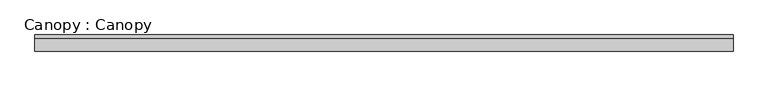
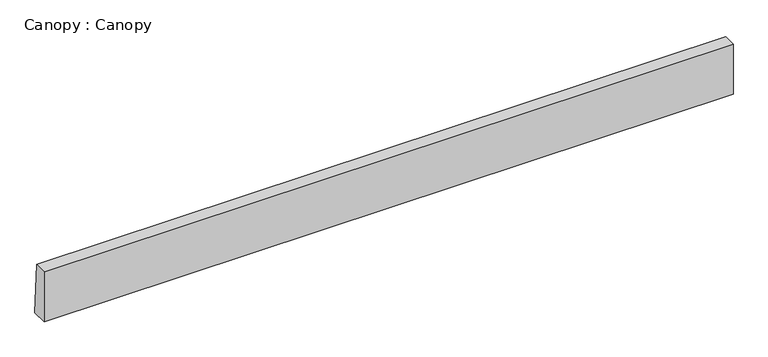
"""IFC4 building model written with IfcOpenShell, lengths in millimetres: proxy geometry, Canopy : Canopy."""

from ifc_helpers import new_model, si_unit, frame, origin, place, context, project, spatial, polyline, outline, extrude, source, transform, mapped, element, save


def canopy_canopy_d66d4a18(model_context):
    return source(origin(), model_context, "Body", "SweptSolid", [
        extrude(outline(polyline([(150.0, 0.0), (0.0, 0.0), (0.0, 500.0), (120.0, 500.0), (150.0, 0.0)])), frame((-3250.0, 0.0, 0.0), z_axis=(1.0, 0.0, 0.0), x_axis=(0.0, 1.0, 0.0)), (0.0, 0.0, 1.0), 6500.0),
    ])


if __name__ == "__main__":
    model = new_model("IFC4")
    model_context = context("Model", 3, world=origin())
    ifc_project = project(units=[si_unit("LENGTHUNIT", "METRE", prefix="MILLI")], contexts=[model_context])
    site = spatial("IfcSite", under=ifc_project)
    building = spatial("IfcBuilding", under=site)
    placement = place(None, origin())
    canopy_canopy_shape = canopy_canopy_d66d4a18(model_context)
    element("IfcBuildingElementProxy", 1, Name="Canopy : Canopy", ObjectType="Canopy : Canopy", at=placement, inside=building, context=model_context, shape_type="MappedRepresentation", body=[
        mapped(canopy_canopy_shape, transform((0.0, 0.0, 0.0), x_axis=(1.0, 0.0, 0.0), y_axis=(0.0, 1.0, 0.0), z_axis=(0.0, 0.0, 1.0))),
    ])
    save(model, "model.ifc")

# Revit data of these elements
# Type "Canopy : Canopy"
#   Type Comments = "CV-AG"
#   H_Rebar Ratio = 0.1
#   Canopy Width [instance default] = 1700 mm
#   Canopy Length [instance default] = 1000 mm
#   Canopy L.P = 120 mm
#   Canopy H.P = 150 mm
#   구조재료 = Concrete_f'c=28MPa(Cylender)
#   Default Elevation = 0
# Element 1 (IfcBuildingElementProxy, "Canopy : Canopy")
#   Canopy Width = 6500 mm
#   Canopy Length = 500 mm
#   Materials on its faces: "Concrete_f'c=28MPa(Cylender)"
# Materials
#   "Concrete_f'c=28MPa(Cylender)": class "Concrete", colour RGB 176 176 176, transparency 0, Description = "Reinf. Conc.", Cost = 0, Image = Concrete.Cast-In-Place.Flat.Polished.Grey.jpg
